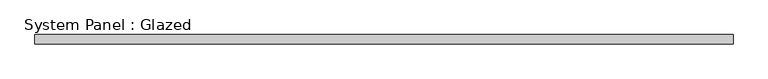
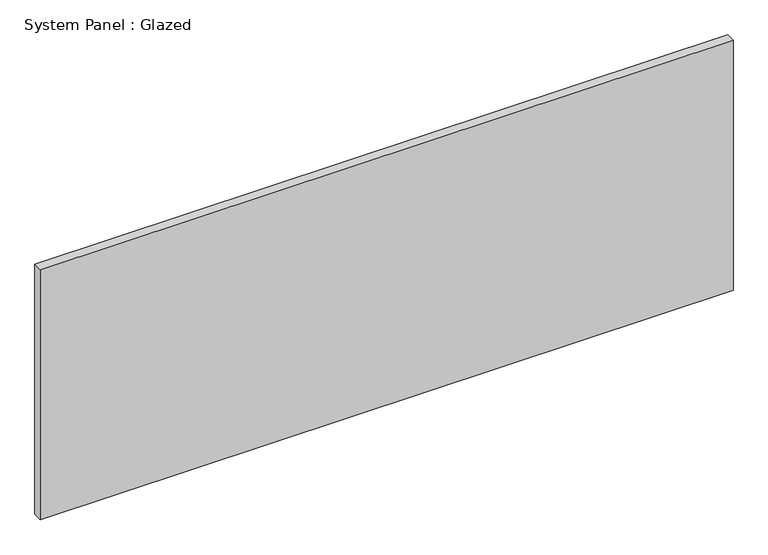
"""IFC4 building model written with IfcOpenShell, lengths in millimetres: plate geometry, System Panel : Glazed."""

from ifc_helpers import new_model, si_unit, origin, origin_with_axes, place, context, project, spatial, polyline, outline, extrude, source, transform, mapped, element, save


def system_panel_glazed_b9c86dac(model_context):
    return source(origin(), model_context, "Body", "SweptSolid", [
        extrude(outline(polyline([(949.9999998, 24.5), (-949.9999998, 24.5), (-949.9999998, 49.5), (949.9999998, 49.5), (949.9999998, 24.5)])), origin_with_axes(), (0.0, 0.0, 1.0), 725.0),
    ])


if __name__ == "__main__":
    model = new_model("IFC4")
    model_context = context("Model", 3, world=origin())
    ifc_project = project(units=[si_unit("LENGTHUNIT", "METRE", prefix="MILLI")], contexts=[model_context])
    site = spatial("IfcSite", under=ifc_project)
    building = spatial("IfcBuilding", under=site)
    placement = place(None, origin())
    system_panel_glazed_shape = system_panel_glazed_b9c86dac(model_context)
    element("IfcPlate", 1, ObjectType="System Panel : Glazed", at=placement, inside=building, context=model_context, shape_type="MappedRepresentation", body=[
        mapped(system_panel_glazed_shape, transform((0.0, 0.0, 0.0), x_axis=(1.0, 0.0, 0.0), y_axis=(0.0, 1.0, 0.0), z_axis=(0.0, 0.0, 1.0))),
    ])
    save(model, "model.ifc")

# Revit data of these elements
# Element 1 (IfcPlate, "System Panel : Glazed")
#   Materials on its faces: "Glass"
# Materials
#   "Glass": class "Glass", colour RGB 0 128 192, transparency 0.9
